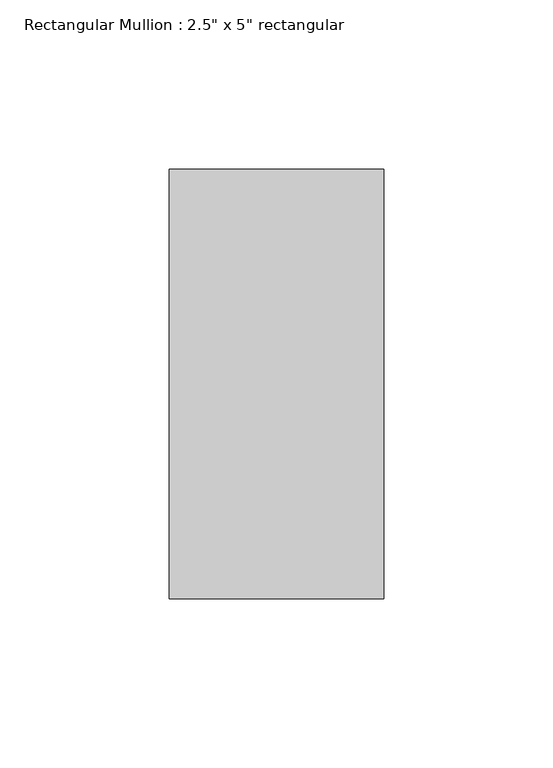
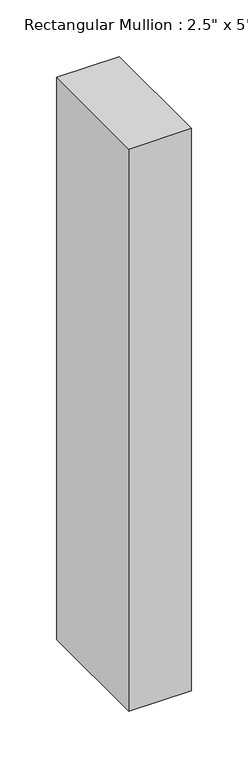
"""IFC4 building model written with IfcOpenShell, lengths in millimetres: member geometry."""

from ifc_helpers import new_model, si_unit, frame, origin, place, context, project, spatial, polyline, outline, extrude, source, transform, mapped, element, save


def member_2e799b37(model_context):
    return source(origin(), model_context, "Body", "SweptSolid", [
        extrude(outline(polyline([(0.0, 63.5), (0.0, -63.5), (-63.5, -63.5), (-63.5, 63.5), (0.0, 63.5)])), frame((0.0, 0.0, -604.75), z_axis=(0.0, 0.0, 1.0), x_axis=(1.0, 0.0, 0.0)), (0.0, 0.0, 1.0), 604.75),
    ])


if __name__ == "__main__":
    model = new_model("IFC4")
    model_context = context("Model", 3, world=origin())
    ifc_project = project(units=[si_unit("LENGTHUNIT", "METRE", prefix="MILLI")], contexts=[model_context])
    site = spatial("IfcSite", under=ifc_project)
    building = spatial("IfcBuilding", under=site)
    placement = place(None, origin())
    member_shape = member_2e799b37(model_context)
    element("IfcMember", 1, ObjectType="Rectangular Mullion : 2.5\" x 5\" rectangular", at=placement, inside=building, context=model_context, shape_type="MappedRepresentation", body=[
        mapped(member_shape, transform((0.0, 0.0, 0.0), x_axis=(1.0, 0.0, 0.0), y_axis=(0.0, 1.0, 0.0), z_axis=(0.0, 0.0, 1.0))),
    ])
    save(model, "model.ifc")

# Revit data of these elements
# Type "Rectangular Mullion : 2.5\" x 5\" rectangular"
#   built-in parameter 1007304 = 0.416667 (stored number, unit not read)
#   built-in parameter 1007301 = 0.104167 (stored number, unit not read)
#   built-in parameter 1007300 = 0.104167 (stored number, unit not read)
# Element 1 (IfcMember, "Rectangular Mullion : 2.5\" x 5\" rectangular")
#   Materials on its faces: "Metal - Aluminum 2"
# Materials
#   "Metal - Aluminum 2": class "Metal", colour RGB 189 187 185, transparency 0
